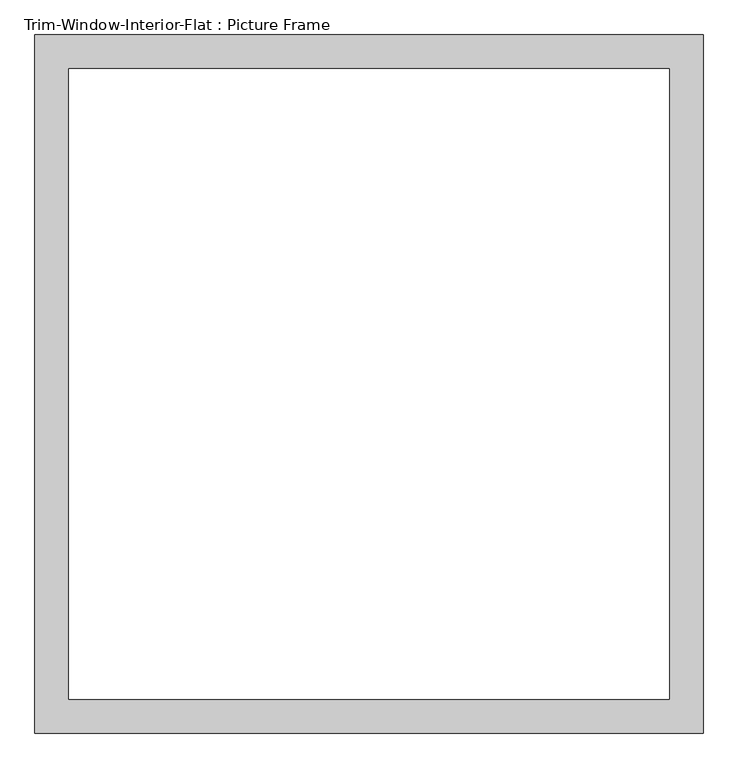
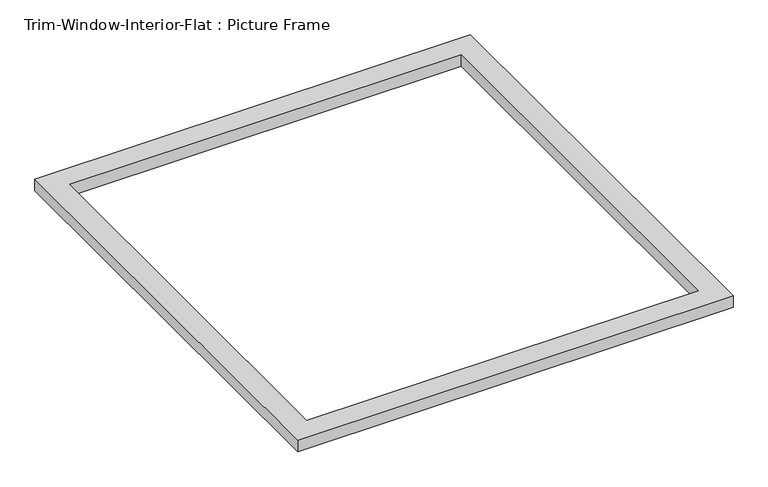
"""IFC4 building model written with IfcOpenShell, lengths in millimetres: proxy geometry, Trim-Window-Interior-Flat : Picture Frame."""

from ifc_helpers import new_model, si_unit, origin, origin_with_axes, place, context, project, spatial, polyline, outline, extrude, source, transform, mapped, element, save


def trim_window_interior_flat_picture_frame_d507ee0b(model_context):
    return source(origin(), model_context, "Body", "SweptSolid", [
        extrude(outline(polyline([(565.15, -44.45), (-565.15, -44.45), (-565.15, 1136.65), (565.15, 1136.65), (565.15, -44.45)]), holes=[polyline([(508.0, 12.7), (508.0, 1079.5), (-508.0, 1079.5), (-508.0, 12.7), (508.0, 12.7)])]), origin_with_axes(), (0.0, 0.0, 1.0), 31.75),
    ])


if __name__ == "__main__":
    model = new_model("IFC4")
    model_context = context("Model", 3, world=origin())
    ifc_project = project(units=[si_unit("LENGTHUNIT", "METRE", prefix="MILLI")], contexts=[model_context])
    site = spatial("IfcSite", under=ifc_project)
    building = spatial("IfcBuilding", under=site)
    placement = place(None, origin())
    trim_window_interior_flat_picture_frame_shape = trim_window_interior_flat_picture_frame_d507ee0b(model_context)
    element("IfcBuildingElementProxy", 1, Name="Trim-Window-Interior-Flat : Picture Frame", ObjectType="Trim-Window-Interior-Flat : Picture Frame", at=placement, inside=building, context=model_context, shape_type="MappedRepresentation", body=[
        mapped(trim_window_interior_flat_picture_frame_shape, transform((0.0, 0.0, 0.0), x_axis=(1.0, 0.0, 0.0), y_axis=(0.0, 1.0, 0.0), z_axis=(0.0, 0.0, 1.0))),
    ])
    save(model, "model.ifc")

# Revit data of these elements
# Type "Trim-Window-Interior-Flat : Picture Frame"
#   Trim Thickness_Picture Frame = 0' - 1 1/4"
#   Trim Width = 0' - 2 1/4"
#   Trim Thickness_with Sill = 0' - 0 3/4"
#   Sill Thickness = 0' - 1 1/4"
#   Opening Width [instance default] = 2' - 0"
#   Opening Height [instance default] = 3' - 0"
#   Default Elevation = 4' - 0"
#   Sill = no
#   Picture Frame = yes
#   Trim Material [instance default] = none
# Element 1 (IfcBuildingElementProxy, "Trim-Window-Interior-Flat : Picture Frame")
#   Opening Width = 3' - 5"
#   Opening Height = 3' - 7"
#   Trim Material = Wood - Stained
#   Materials on its faces: "Wood - Stained"
# Materials
#   "Wood - Stained": class "Wood", colour RGB 224 178 126, transparency 0, Cost = 0
